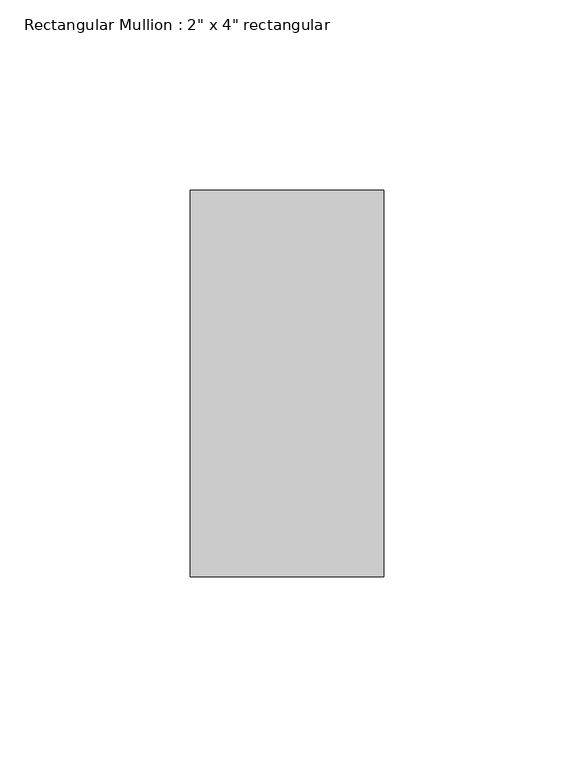
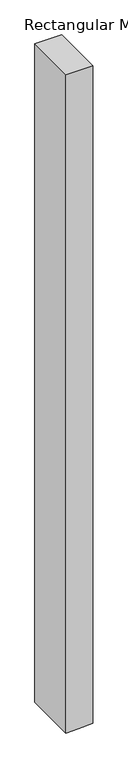
"""IFC4 building model written with IfcOpenShell, lengths in millimetres: member geometry."""

import ifcopenshell
import ifcopenshell.guid

model = None  # the IFC model being written
_history = None  # IfcOwnerHistory: only IFC2X3 demands one
_inside = {}  # id of a spatial element -> (the spatial element, [elements in it])
_under = {}  # id of a project, library or spatial element -> (it, [spatial elements below it])
_declared = {}  # id of a project -> (the project, [libraries it declares])
_typed = {}  # id of a type object -> (the type object, [elements of that type])
_made_of = {}  # id of a material, layer set ... -> (it, [elements and type objects made of it])


def new_model(schema):
    """Start an empty IFC model of exactly this schema.

    Asked for "IFC4X3", IfcOpenShell would pick the latest addendum, in which some entities
    have other attributes; the version numbers below select the first issue.
    IFC2X3 requires an IfcOwnerHistory on every rooted entity: one is made here for all.
    """
    global model, _history
    if schema == "IFC4X3":
        model = ifcopenshell.file(schema_version=(4, 3, 0, 0))
    else:
        model = ifcopenshell.file(schema=schema)
    _inside.clear()
    _under.clear()
    _declared.clear()
    _typed.clear()
    _made_of.clear()
    _history = None
    if model.schema == "IFC2X3":
        org = make("IfcOrganization", Name="unknown")
        user = make(
            "IfcPersonAndOrganization",
            ThePerson=make("IfcPerson", FamilyName="unknown"),
            TheOrganization=org,
        )
        app = make(
            "IfcApplication",
            ApplicationDeveloper=org,
            Version="unknown",
            ApplicationFullName="unknown",
            ApplicationIdentifier="unknown",
        )
        _history = make(
            "IfcOwnerHistory",
            OwningUser=user,
            OwningApplication=app,
            ChangeAction="ADDED",
            CreationDate=0,
        )
    return model


def make(cls, **values):
    """One entity of the class cls with the attributes given. An attribute that is None is left unset."""
    return model.create_entity(
        cls, **{name: value for name, value in values.items() if value is not None}
    )


def rooted(cls, **values):
    """An entity with a GlobalId (a new one), such as an element, a storey or a relation."""
    return make(cls, GlobalId=ifcopenshell.guid.new(), OwnerHistory=_history, **values)


def si_unit(unit_type, name, prefix=None):
    """IfcSIUnit, for example si_unit("LENGTHUNIT", "METRE", prefix="MILLI")."""
    return make("IfcSIUnit", UnitType=unit_type, Prefix=prefix, Name=name)


def assignment(units):
    """IfcUnitAssignment: the units of a project."""
    return None if units is None else make("IfcUnitAssignment", Units=units)


def point(xyz):
    """IfcCartesianPoint."""
    return None if xyz is None else make("IfcCartesianPoint", Coordinates=xyz)


def direction(xyz):
    """IfcDirection."""
    return None if xyz is None else make("IfcDirection", DirectionRatios=xyz)


def frame(location, z_axis=None, x_axis=None):
    """IfcAxis2Placement3D, a coordinate frame: its origin and axes. An axis left out is left unset."""
    return make(
        "IfcAxis2Placement3D",
        Location=point(location),
        Axis=direction(z_axis),
        RefDirection=direction(x_axis),
    )


def origin():
    """The frame at (0, 0, 0) with its axes left unset."""
    return frame((0.0, 0.0, 0.0))


def place(relative_to, where):
    """IfcLocalPlacement: puts the frame where relative to a parent placement (None: the world)."""
    return make(
        "IfcLocalPlacement", PlacementRelTo=relative_to, RelativePlacement=where
    )


def context(
    kind, dimensions, precision=None, world=None, true_north=None, identifier=None
):
    """IfcGeometricRepresentationContext, for example the 3D "Model" context."""
    return make(
        "IfcGeometricRepresentationContext",
        ContextIdentifier=identifier,
        ContextType=kind,
        CoordinateSpaceDimension=dimensions,
        Precision=precision,
        WorldCoordinateSystem=world,
        TrueNorth=true_north,
    )


def project(units=None, contexts=None):
    """IfcProject with its units and contexts."""
    return rooted(
        "IfcProject",
        Name="project",
        RepresentationContexts=contexts,
        UnitsInContext=assignment(units),
    )


def spatial(cls, under=None, at=None, **own):
    """A site, building, storey or space (cls), placed at a placement, below another one or the project."""
    s = rooted(cls, ObjectPlacement=at, **own)
    if under is not None:
        _under.setdefault(under.id(), (under, []))[1].append(s)
    return s


def polyline(points):
    """IfcPolyline through the points."""
    return make("IfcPolyline", Points=[point(p) for p in points])


def outline(outer, holes=None, kind="AREA"):
    """IfcArbitraryClosedProfileDef: a profile drawn as a closed curve; with holes, ...WithVoids."""
    if holes is None:
        return make("IfcArbitraryClosedProfileDef", ProfileType=kind, OuterCurve=outer)
    return make(
        "IfcArbitraryProfileDefWithVoids",
        ProfileType=kind,
        OuterCurve=outer,
        InnerCurves=holes,
    )


def extrude(swept, where, along, depth):
    """IfcExtrudedAreaSolid: the profile swept, set in the frame where, extruded along a direction by depth."""
    return make(
        "IfcExtrudedAreaSolid",
        SweptArea=swept,
        Position=where,
        ExtrudedDirection=direction(along),
        Depth=depth,
    )


def shape(context_of_items, identifier, shape_type, items):
    """IfcShapeRepresentation: the items that make up one representation, for example the "Body"."""
    return make(
        "IfcShapeRepresentation",
        ContextOfItems=context_of_items,
        RepresentationIdentifier=identifier,
        RepresentationType=shape_type,
        Items=items,
    )


def source(mapping_origin, context_of_items, identifier, shape_type, items):
    """IfcRepresentationMap: a shape defined once, which mapped items show again and again."""
    return make(
        "IfcRepresentationMap",
        MappingOrigin=mapping_origin,
        MappedRepresentation=shape(context_of_items, identifier, shape_type, items),
    )


def transform(
    local_origin,
    x_axis=None,
    y_axis=None,
    z_axis=None,
    scale=None,
    scale2=None,
    scale3=None,
    uniform=True,
):
    """IfcCartesianTransformationOperator3D, or its non-uniform kind. x_axis, y_axis, z_axis: its Axis1, 2, 3."""
    if uniform:
        return make(
            "IfcCartesianTransformationOperator3D",
            Axis1=direction(x_axis),
            Axis2=direction(y_axis),
            LocalOrigin=point(local_origin),
            Scale=scale,
            Axis3=direction(z_axis),
        )
    return make(
        "IfcCartesianTransformationOperator3DnonUniform",
        Axis1=direction(x_axis),
        Axis2=direction(y_axis),
        LocalOrigin=point(local_origin),
        Scale=scale,
        Axis3=direction(z_axis),
        Scale2=scale2,
        Scale3=scale3,
    )


def mapped(mapping_source, mapping_target):
    """IfcMappedItem: shows the shape of a source again, moved by a transform."""
    return make(
        "IfcMappedItem", MappingSource=mapping_source, MappingTarget=mapping_target
    )


def made_of(thing, what):
    """Note that an element or type object is made of a material, layer set ...; save() writes the relation."""
    if what is not None:
        _made_of.setdefault(what.id(), (what, []))[1].append(thing)
    return thing


def element(
    cls,
    number,
    at=None,
    inside=None,
    cuts=None,
    type_object=None,
    material=None,
    context=None,
    identifier="Body",
    shape_type=None,
    held_by="IfcProductDefinitionShape",
    body=None,
    shapes=None,
    **own,
):
    """One element of the class cls, such as IfcWall. Its Tag is "e" and its number.

    at: its placement. inside: the storey or other place that contains it. cuts: it is an
    opening in that element (IfcRelVoidsElement). A single representation is given by context,
    identifier, shape_type and body (its items); several are given by shapes. held_by: the class
    of the entity that holds the representations. save() writes the other relations.
    """
    e = rooted(cls, Tag="e%d" % number, ObjectPlacement=at, **own)
    if body is not None:
        shapes = [shape(context, identifier, shape_type, body)]
    if shapes is not None:
        e.Representation = make(held_by, Representations=shapes)
    if inside is not None:
        _inside.setdefault(inside.id(), (inside, []))[1].append(e)
    if cuts is not None:
        rooted(
            "IfcRelVoidsElement", RelatingBuildingElement=cuts, RelatedOpeningElement=e
        )
    if type_object is not None:
        _typed.setdefault(type_object.id(), (type_object, []))[1].append(e)
    return made_of(e, material)


def aggregate(whole, parts):
    """IfcRelAggregates: a whole, such as a stair, and the parts it consists of."""
    return rooted("IfcRelAggregates", RelatingObject=whole, RelatedObjects=parts)


def save(model, path):
    """Write the relations noted so far, then the file.

    IfcRelAggregates (storeys below a building ...), IfcRelContainedInSpatialStructure (elements
    in a storey), IfcRelDefinesByType, IfcRelAssociatesMaterial and IfcRelDeclares: one each for
    every whole, place, type object, material and project.
    """
    for whole, parts in _under.values():
        aggregate(whole, parts)
    for where, things in _inside.values():
        rooted(
            "IfcRelContainedInSpatialStructure",
            RelatedElements=things,
            RelatingStructure=where,
        )
    for kind, things in _typed.values():
        rooted("IfcRelDefinesByType", RelatedObjects=things, RelatingType=kind)
    for what, things in _made_of.values():
        rooted("IfcRelAssociatesMaterial", RelatedObjects=things, RelatingMaterial=what)
    for by, libraries in _declared.values():
        rooted("IfcRelDeclares", RelatingContext=by, RelatedDefinitions=libraries)
    model.write(path)


def member_c2cb099a(model_context):
    return source(origin(), model_context, "Body", "SweptSolid", [
        extrude(outline(polyline([(0.0, 25.4), (0.0, -25.4), (-1318.3022126, -25.4), (-1317.3319972, -2.1148317), (-1316.1855459, 25.4), (0.0, 25.4)])), frame((0.0, -50.8, 0.0), z_axis=(0.0, 1.0, 0.0), x_axis=(0.0, 0.0, 1.0)), (0.0, 0.0, 1.0), 101.6),
    ])


if __name__ == "__main__":
    model = new_model("IFC4")
    model_context = context("Model", 3, world=origin())
    ifc_project = project(units=[si_unit("LENGTHUNIT", "METRE", prefix="MILLI")], contexts=[model_context])
    site = spatial("IfcSite", under=ifc_project)
    building = spatial("IfcBuilding", under=site)
    placement = place(None, origin())
    member_shape = member_c2cb099a(model_context)
    element("IfcMember", 1, ObjectType="Rectangular Mullion : 2\" x 4\" rectangular", at=placement, inside=building, context=model_context, shape_type="MappedRepresentation", body=[
        mapped(member_shape, transform((0.0, 0.0, 0.0), x_axis=(1.0, 0.0, 0.0), y_axis=(0.0, 1.0, 0.0), z_axis=(0.0, 0.0, 1.0))),
    ])
    save(model, "model.ifc")

# Revit data of these elements
# Type "Rectangular Mullion : 2\" x 4\" rectangular"
#   built-in parameter 1007304 = 0.333333 (stored number, unit not read)
#   built-in parameter 1007301 = 0.0833333 (stored number, unit not read)
#   built-in parameter 1007300 = 0.0833333 (stored number, unit not read)
# Element 1 (IfcMember, "Rectangular Mullion : 2\" x 4\" rectangular")
#   Materials on its faces: "PAINTED STEEL C CHANNEL"
# Materials
#   "PAINTED STEEL C CHANNEL": class "Generic", colour RGB 88 62 61, transparency 0, Cost = 0
